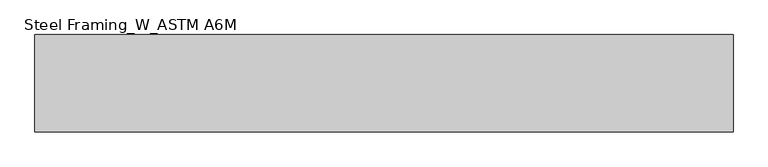
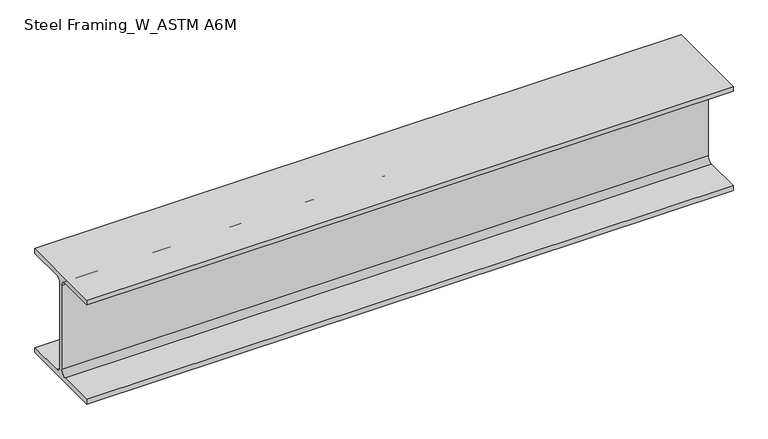
"""IFC4 building model written with IfcOpenShell, lengths in millimetres: beam geometry, Steel Framing_W_ASTM A6M : H_SB_AR_S02_W250x49.1_G5."""

from ifc_helpers import new_model, si_unit, point, frame, frame_2d, origin, place, context, project, spatial, polyline, circle_curve, trimmed, segment, composite_curve, outline, extrude, source, transform, mapped, element, save


def steel_framing_w_astm_a6m_ee6b765e(model_context):
    return source(origin(), model_context, "Body", "SweptSolid", [
        extrude(outline(composite_curve([segment(polyline([(101.0, -112.5), (101.0, -123.5), (-101.0, -123.5), (-101.0, -112.5), (-16.385, -112.5)]), True, "CONTINUOUS"), segment(trimmed(circle_curve(frame_2d((-16.385, -99.8)), 12.7), [point((-16.385, -112.5))], [point((-3.685, -99.8))], True, "CARTESIAN"), True, "CONTINUOUS"), segment(polyline([(-3.685, -99.8), (-3.685, 99.8)]), True, "CONTINUOUS"), segment(trimmed(circle_curve(frame_2d((-16.385, 99.8)), 12.7), [point((-3.685, 99.8))], [point((-16.385, 112.5))], True, "CARTESIAN"), True, "CONTINUOUS"), segment(polyline([(-16.385, 112.5), (-101.0, 112.5), (-101.0, 123.5), (101.0, 123.5), (101.0, 112.5), (16.385, 112.5)]), True, "CONTINUOUS"), segment(trimmed(circle_curve(frame_2d((16.385, 99.8)), 12.7), [point((16.385, 112.5))], [point((3.685, 99.8))], True, "CARTESIAN"), True, "CONTINUOUS"), segment(polyline([(3.685, 99.8), (3.685, -99.8)]), True, "CONTINUOUS"), segment(trimmed(circle_curve(frame_2d((16.385, -99.8)), 12.7), [point((3.685, -99.8))], [point((16.385, -112.5))], True, "CARTESIAN"), True, "CONTINUOUS"), segment(polyline([(16.385, -112.5), (101.0, -112.5)]), True, "CONTINUOUS")], self_intersect=False)), frame((-634.3, 0.0, 0.0), z_axis=(1.0, 0.0, 0.0), x_axis=(0.0, 1.0, 0.0)), (0.0, 0.0, 1.0), 1451.3),
    ])


if __name__ == "__main__":
    model = new_model("IFC4")
    model_context = context("Model", 3, world=origin())
    ifc_project = project(units=[si_unit("LENGTHUNIT", "METRE", prefix="MILLI")], contexts=[model_context])
    site = spatial("IfcSite", under=ifc_project)
    building = spatial("IfcBuilding", under=site)
    placement = place(None, origin())
    steel_framing_w_astm_a6m_shape = steel_framing_w_astm_a6m_ee6b765e(model_context)
    element("IfcBeam", 1, ObjectType="Steel Framing_W_ASTM A6M : H_SB_AR_S02_W250x49.1_G5", at=placement, inside=building, context=model_context, shape_type="MappedRepresentation", body=[
        mapped(steel_framing_w_astm_a6m_shape, transform((0.0, 0.0, 0.0), x_axis=(1.0, 0.0, 0.0), y_axis=(0.0, 1.0, 0.0), z_axis=(0.0, 0.0, 1.0))),
    ])
    save(model, "model.ifc")

# Revit data of these elements
# Type "Steel Framing_W_ASTM A6M : H_SB_AR_S02_W250x49.1_G5"
#   Type Mark = "G5"
#   Section Name Key = "W10x33"
#   Width = 20.2 cm
#   Web Thickness = 0.737 cm
#   Web Fillet = 1.27 cm
#   Warping Constant = 212000.0 cm⁶
#   Torsional Moment of Inertia = 24.30 cm⁴
#   Section Area = 62.6 cm²
#   Plastic Modulus weak axis = 229.0 cm³
#   Plastic Modulus strong axis = 636.0 cm³
#   Perimeter = 1.27 m²/m
#   Nominal Weight = 49.10 kgf/m
#   Moment of Inertia weak axis = 1520.00 cm⁴
#   Moment of Inertia strong axis = 7120.00 cm⁴
#   Height = 24.7 cm
#   Flange Thickness = 1.1 cm
#   Elastic Modulus weak axis = 151.0 cm³
#   Elastic Modulus strong axis = 574.0 cm³
#   Centroid Vertical = 12.35 cm
#   Centroid Horizontal = 10.1 cm
#   Length [instance default] = 1500 mm
#   Structural Material [instance default] = Steel, 45-345
#   Bolt Spacing = 0
#   Assembly Code = ""
# Element 1 (IfcBeam, "Steel Framing_W_ASTM A6M : H_SB_AR_S02_W250x49.1_G5")
#   Materials on its faces: "Steel, 45-345"
# Materials
#   "Steel, 45-345": class "Metal", colour RGB 189 187 185, transparency 0, Description = "Steel 345 MPa", Cost = 0
